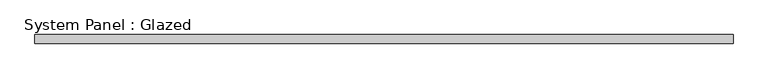
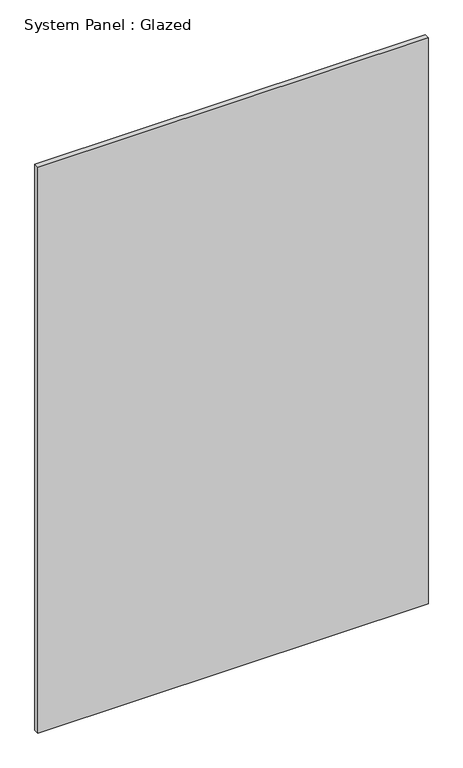
"""IFC4 building model written with IfcOpenShell, lengths in millimetres: plate geometry, System Panel : Glazed."""

from ifc_helpers import new_model, si_unit, origin, origin_with_axes, place, context, project, spatial, polyline, outline, extrude, source, transform, mapped, element, save


def system_panel_glazed_cab7de13(model_context):
    return source(origin(), model_context, "Body", "SweptSolid", [
        extrude(outline(polyline([(961.6833335, 24.5), (-961.6833335, 24.5), (-961.6833335, 49.5), (961.6833335, 49.5), (961.6833335, 24.5)])), origin_with_axes(), (0.0, 0.0, 1.0), 2950.0),
    ])


if __name__ == "__main__":
    model = new_model("IFC4")
    model_context = context("Model", 3, world=origin())
    ifc_project = project(units=[si_unit("LENGTHUNIT", "METRE", prefix="MILLI")], contexts=[model_context])
    site = spatial("IfcSite", under=ifc_project)
    building = spatial("IfcBuilding", under=site)
    placement = place(None, origin())
    system_panel_glazed_shape = system_panel_glazed_cab7de13(model_context)
    element("IfcPlate", 1, ObjectType="System Panel : Glazed", at=placement, inside=building, context=model_context, shape_type="MappedRepresentation", body=[
        mapped(system_panel_glazed_shape, transform((0.0, 0.0, 0.0), x_axis=(1.0, 0.0, 0.0), y_axis=(0.0, 1.0, 0.0), z_axis=(0.0, 0.0, 1.0))),
    ])
    save(model, "model.ifc")

# Revit data of these elements
# Element 1 (IfcPlate, "System Panel : Glazed")
#   Materials on its faces: "Glass"
# Materials
#   "Glass": class "Glass", colour RGB 0 128 192, transparency 0.9
